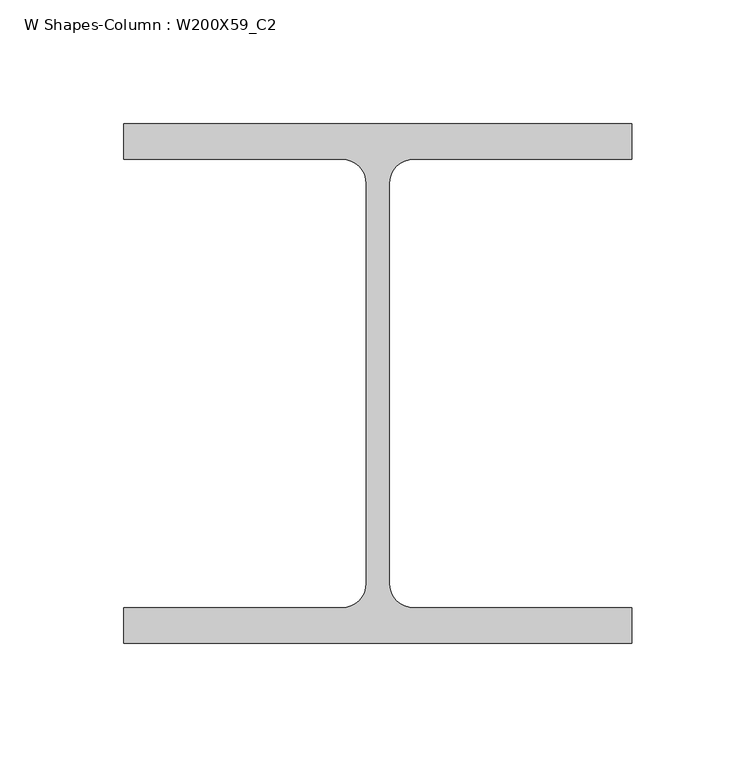
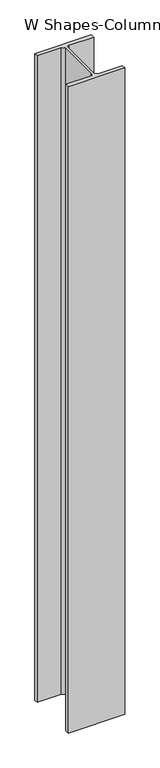
"""IFC4 building model written with IfcOpenShell, lengths in millimetres: column geometry, W Shapes-Column : W200X59_C2."""

from ifc_helpers import new_model, si_unit, point, frame, frame_2d, origin, place, context, project, spatial, polyline, circle_curve, trimmed, segment, composite_curve, outline, extrude, source, transform, mapped, element, save


def w_shapes_column_w200x59_c2_7c440a81(model_context):
    return source(origin(), model_context, "Body", "SweptSolid", [
        extrude(outline(composite_curve([segment(polyline([(102.489, 104.775), (102.489, 90.551), (14.5796, 90.551)]), True, "CONTINUOUS"), segment(trimmed(circle_curve(frame_2d((14.5796, 80.5434)), 10.0076), [point((14.5796, 90.551))], [point((4.572, 80.5434))], True, "CARTESIAN"), True, "CONTINUOUS"), segment(polyline([(4.572, 80.5434), (4.572, -80.5434)]), True, "CONTINUOUS"), segment(trimmed(circle_curve(frame_2d((14.5796, -80.5434)), 10.0076), [point((4.572, -80.5434))], [point((14.5796, -90.551))], True, "CARTESIAN"), True, "CONTINUOUS"), segment(polyline([(14.5796, -90.551), (102.489, -90.551), (102.489, -104.775), (-102.489, -104.775), (-102.489, -90.551), (-14.5796, -90.551)]), True, "CONTINUOUS"), segment(trimmed(circle_curve(frame_2d((-14.5796, -80.5434)), 10.0076), [point((-14.5796, -90.551))], [point((-4.572, -80.5434))], True, "CARTESIAN"), True, "CONTINUOUS"), segment(polyline([(-4.572, -80.5434), (-4.572, 80.5434)]), True, "CONTINUOUS"), segment(trimmed(circle_curve(frame_2d((-14.5796, 80.5434)), 10.0076), [point((-4.572, 80.5434))], [point((-14.5796, 90.551))], True, "CARTESIAN"), True, "CONTINUOUS"), segment(polyline([(-14.5796, 90.551), (-102.489, 90.551), (-102.489, 104.775), (102.489, 104.775)]), True, "CONTINUOUS")], self_intersect=False)), frame((0.0, 0.0, 6546.0), z_axis=(0.0, 0.0, 1.0), x_axis=(1.0, 0.0, 0.0)), (0.0, 0.0, 1.0), 2484.0),
    ])


if __name__ == "__main__":
    model = new_model("IFC4")
    model_context = context("Model", 3, world=origin())
    ifc_project = project(units=[si_unit("LENGTHUNIT", "METRE", prefix="MILLI")], contexts=[model_context])
    site = spatial("IfcSite", under=ifc_project)
    building = spatial("IfcBuilding", under=site)
    placement = place(None, origin())
    w_shapes_column_w200x59_c2_shape = w_shapes_column_w200x59_c2_7c440a81(model_context)
    element("IfcColumn", 1, ObjectType="W Shapes-Column : W200X59_C2", at=placement, inside=building, context=model_context, shape_type="MappedRepresentation", body=[
        mapped(w_shapes_column_w200x59_c2_shape, transform((0.0, 0.0, 0.0), x_axis=(1.0, 0.0, 0.0), y_axis=(0.0, 1.0, 0.0), z_axis=(0.0, 0.0, 1.0))),
    ])
    save(model, "model.ifc")

# Revit data of these elements
# Type "W Shapes-Column : W200X59_C2"
#   Section Name Key = "W8x40"
#   Assembly Code = "B10"
#   Width = 20.4978 cm
#   Web Thickness = 0.9144 cm
#   Web Fillet = 1.0008 cm
#   Warping Constant = 194957.0 cm⁶
#   Torsional Moment of Inertia = 46.6179 cm⁴
#   Section Area = 75.4837 cm²
#   Plastic Modulus weak axis = 303.161 cm³
#   Plastic Modulus strong axis = 652.205 cm³
#   Perimeter = 1.20396 m²/m
#   Nominal Weight = 59.5266 kgf/m
#   Moment of Inertia weak axis = 2043.70 cm⁴
#   Moment of Inertia strong axis = 6076.98 cm⁴
#   Height = 20.955 cm
#   Flange Thickness = 1.4224 cm
#   Elastic Modulus weak axis = 199.922 cm³
#   Elastic Modulus strong axis = 581.741 cm³
#   Clear Web Height = 19.05 cm
#   Centroid Vertical = 10.4775 cm
#   Centroid Horizontal = 10.2489 cm
#   Bolt Spacing = 13.97 cm
#   Structural Material [instance default] = Steel ASTM A992
#   Principal Axes Angle = 0
# Element 1 (IfcColumn, "W Shapes-Column : W200X59_C2")
#   Structural Material = none
# Materials
#   "Steel ASTM A992": class "Metal", colour RGB 199 199 199, transparency 0, Description = "Structural steel 50ksi", Cost = 0
